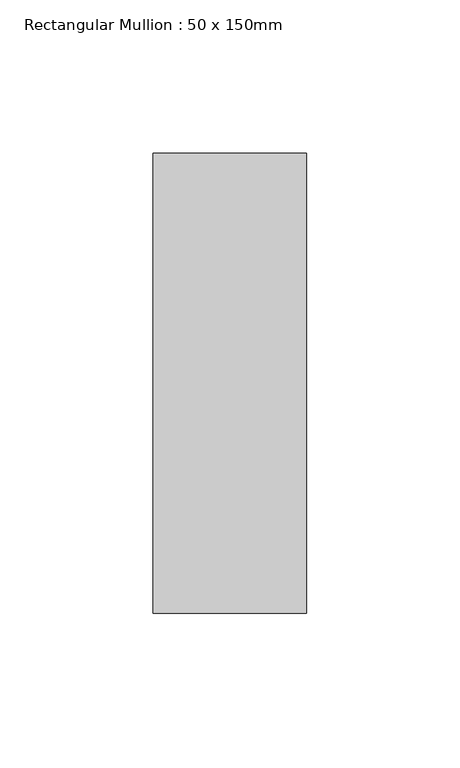
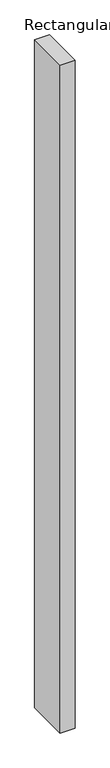
"""IFC4 building model written with IfcOpenShell, lengths in millimetres: member geometry, Rectangular Mullion : 50 x 150mm."""

import ifcopenshell
import ifcopenshell.guid

model = None  # the IFC model being written
_history = None  # IfcOwnerHistory: only IFC2X3 demands one
_inside = {}  # id of a spatial element -> (the spatial element, [elements in it])
_under = {}  # id of a project, library or spatial element -> (it, [spatial elements below it])
_declared = {}  # id of a project -> (the project, [libraries it declares])
_typed = {}  # id of a type object -> (the type object, [elements of that type])
_made_of = {}  # id of a material, layer set ... -> (it, [elements and type objects made of it])


def new_model(schema):
    """Start an empty IFC model of exactly this schema.

    Asked for "IFC4X3", IfcOpenShell would pick the latest addendum, in which some entities
    have other attributes; the version numbers below select the first issue.
    IFC2X3 requires an IfcOwnerHistory on every rooted entity: one is made here for all.
    """
    global model, _history
    if schema == "IFC4X3":
        model = ifcopenshell.file(schema_version=(4, 3, 0, 0))
    else:
        model = ifcopenshell.file(schema=schema)
    _inside.clear()
    _under.clear()
    _declared.clear()
    _typed.clear()
    _made_of.clear()
    _history = None
    if model.schema == "IFC2X3":
        org = make("IfcOrganization", Name="unknown")
        user = make(
            "IfcPersonAndOrganization",
            ThePerson=make("IfcPerson", FamilyName="unknown"),
            TheOrganization=org,
        )
        app = make(
            "IfcApplication",
            ApplicationDeveloper=org,
            Version="unknown",
            ApplicationFullName="unknown",
            ApplicationIdentifier="unknown",
        )
        _history = make(
            "IfcOwnerHistory",
            OwningUser=user,
            OwningApplication=app,
            ChangeAction="ADDED",
            CreationDate=0,
        )
    return model


def make(cls, **values):
    """One entity of the class cls with the attributes given. An attribute that is None is left unset."""
    return model.create_entity(
        cls, **{name: value for name, value in values.items() if value is not None}
    )


def rooted(cls, **values):
    """An entity with a GlobalId (a new one), such as an element, a storey or a relation."""
    return make(cls, GlobalId=ifcopenshell.guid.new(), OwnerHistory=_history, **values)


def si_unit(unit_type, name, prefix=None):
    """IfcSIUnit, for example si_unit("LENGTHUNIT", "METRE", prefix="MILLI")."""
    return make("IfcSIUnit", UnitType=unit_type, Prefix=prefix, Name=name)


def assignment(units):
    """IfcUnitAssignment: the units of a project."""
    return None if units is None else make("IfcUnitAssignment", Units=units)


def point(xyz):
    """IfcCartesianPoint."""
    return None if xyz is None else make("IfcCartesianPoint", Coordinates=xyz)


def direction(xyz):
    """IfcDirection."""
    return None if xyz is None else make("IfcDirection", DirectionRatios=xyz)


def frame(location, z_axis=None, x_axis=None):
    """IfcAxis2Placement3D, a coordinate frame: its origin and axes. An axis left out is left unset."""
    return make(
        "IfcAxis2Placement3D",
        Location=point(location),
        Axis=direction(z_axis),
        RefDirection=direction(x_axis),
    )


def origin():
    """The frame at (0, 0, 0) with its axes left unset."""
    return frame((0.0, 0.0, 0.0))


def place(relative_to, where):
    """IfcLocalPlacement: puts the frame where relative to a parent placement (None: the world)."""
    return make(
        "IfcLocalPlacement", PlacementRelTo=relative_to, RelativePlacement=where
    )


def context(
    kind, dimensions, precision=None, world=None, true_north=None, identifier=None
):
    """IfcGeometricRepresentationContext, for example the 3D "Model" context."""
    return make(
        "IfcGeometricRepresentationContext",
        ContextIdentifier=identifier,
        ContextType=kind,
        CoordinateSpaceDimension=dimensions,
        Precision=precision,
        WorldCoordinateSystem=world,
        TrueNorth=true_north,
    )


def project(units=None, contexts=None):
    """IfcProject with its units and contexts."""
    return rooted(
        "IfcProject",
        Name="project",
        RepresentationContexts=contexts,
        UnitsInContext=assignment(units),
    )


def spatial(cls, under=None, at=None, **own):
    """A site, building, storey or space (cls), placed at a placement, below another one or the project."""
    s = rooted(cls, ObjectPlacement=at, **own)
    if under is not None:
        _under.setdefault(under.id(), (under, []))[1].append(s)
    return s


def polyline(points):
    """IfcPolyline through the points."""
    return make("IfcPolyline", Points=[point(p) for p in points])


def outline(outer, holes=None, kind="AREA"):
    """IfcArbitraryClosedProfileDef: a profile drawn as a closed curve; with holes, ...WithVoids."""
    if holes is None:
        return make("IfcArbitraryClosedProfileDef", ProfileType=kind, OuterCurve=outer)
    return make(
        "IfcArbitraryProfileDefWithVoids",
        ProfileType=kind,
        OuterCurve=outer,
        InnerCurves=holes,
    )


def extrude(swept, where, along, depth):
    """IfcExtrudedAreaSolid: the profile swept, set in the frame where, extruded along a direction by depth."""
    return make(
        "IfcExtrudedAreaSolid",
        SweptArea=swept,
        Position=where,
        ExtrudedDirection=direction(along),
        Depth=depth,
    )


def shape(context_of_items, identifier, shape_type, items):
    """IfcShapeRepresentation: the items that make up one representation, for example the "Body"."""
    return make(
        "IfcShapeRepresentation",
        ContextOfItems=context_of_items,
        RepresentationIdentifier=identifier,
        RepresentationType=shape_type,
        Items=items,
    )


def source(mapping_origin, context_of_items, identifier, shape_type, items):
    """IfcRepresentationMap: a shape defined once, which mapped items show again and again."""
    return make(
        "IfcRepresentationMap",
        MappingOrigin=mapping_origin,
        MappedRepresentation=shape(context_of_items, identifier, shape_type, items),
    )


def transform(
    local_origin,
    x_axis=None,
    y_axis=None,
    z_axis=None,
    scale=None,
    scale2=None,
    scale3=None,
    uniform=True,
):
    """IfcCartesianTransformationOperator3D, or its non-uniform kind. x_axis, y_axis, z_axis: its Axis1, 2, 3."""
    if uniform:
        return make(
            "IfcCartesianTransformationOperator3D",
            Axis1=direction(x_axis),
            Axis2=direction(y_axis),
            LocalOrigin=point(local_origin),
            Scale=scale,
            Axis3=direction(z_axis),
        )
    return make(
        "IfcCartesianTransformationOperator3DnonUniform",
        Axis1=direction(x_axis),
        Axis2=direction(y_axis),
        LocalOrigin=point(local_origin),
        Scale=scale,
        Axis3=direction(z_axis),
        Scale2=scale2,
        Scale3=scale3,
    )


def mapped(mapping_source, mapping_target):
    """IfcMappedItem: shows the shape of a source again, moved by a transform."""
    return make(
        "IfcMappedItem", MappingSource=mapping_source, MappingTarget=mapping_target
    )


def made_of(thing, what):
    """Note that an element or type object is made of a material, layer set ...; save() writes the relation."""
    if what is not None:
        _made_of.setdefault(what.id(), (what, []))[1].append(thing)
    return thing


def element(
    cls,
    number,
    at=None,
    inside=None,
    cuts=None,
    type_object=None,
    material=None,
    context=None,
    identifier="Body",
    shape_type=None,
    held_by="IfcProductDefinitionShape",
    body=None,
    shapes=None,
    **own,
):
    """One element of the class cls, such as IfcWall. Its Tag is "e" and its number.

    at: its placement. inside: the storey or other place that contains it. cuts: it is an
    opening in that element (IfcRelVoidsElement). A single representation is given by context,
    identifier, shape_type and body (its items); several are given by shapes. held_by: the class
    of the entity that holds the representations. save() writes the other relations.
    """
    e = rooted(cls, Tag="e%d" % number, ObjectPlacement=at, **own)
    if body is not None:
        shapes = [shape(context, identifier, shape_type, body)]
    if shapes is not None:
        e.Representation = make(held_by, Representations=shapes)
    if inside is not None:
        _inside.setdefault(inside.id(), (inside, []))[1].append(e)
    if cuts is not None:
        rooted(
            "IfcRelVoidsElement", RelatingBuildingElement=cuts, RelatedOpeningElement=e
        )
    if type_object is not None:
        _typed.setdefault(type_object.id(), (type_object, []))[1].append(e)
    return made_of(e, material)


def aggregate(whole, parts):
    """IfcRelAggregates: a whole, such as a stair, and the parts it consists of."""
    return rooted("IfcRelAggregates", RelatingObject=whole, RelatedObjects=parts)


def save(model, path):
    """Write the relations noted so far, then the file.

    IfcRelAggregates (storeys below a building ...), IfcRelContainedInSpatialStructure (elements
    in a storey), IfcRelDefinesByType, IfcRelAssociatesMaterial and IfcRelDeclares: one each for
    every whole, place, type object, material and project.
    """
    for whole, parts in _under.values():
        aggregate(whole, parts)
    for where, things in _inside.values():
        rooted(
            "IfcRelContainedInSpatialStructure",
            RelatedElements=things,
            RelatingStructure=where,
        )
    for kind, things in _typed.values():
        rooted("IfcRelDefinesByType", RelatedObjects=things, RelatingType=kind)
    for what, things in _made_of.values():
        rooted("IfcRelAssociatesMaterial", RelatedObjects=things, RelatingMaterial=what)
    for by, libraries in _declared.values():
        rooted("IfcRelDeclares", RelatingContext=by, RelatedDefinitions=libraries)
    model.write(path)


def rectangular_mullion_50_x_150mm_6225e4e3(model_context):
    return source(origin(), model_context, "Body", "SweptSolid", [
        extrude(outline(polyline([(25.0, 75.0), (25.0, -75.0), (-25.0, -75.0), (-25.0, 75.0), (25.0, 75.0)])), frame((0.0, 0.0, -2400.0), z_axis=(0.0, 0.0, 1.0), x_axis=(1.0, 0.0, 0.0)), (0.0, 0.0, 1.0), 2400.0),
    ])


if __name__ == "__main__":
    model = new_model("IFC4")
    model_context = context("Model", 3, world=origin())
    ifc_project = project(units=[si_unit("LENGTHUNIT", "METRE", prefix="MILLI")], contexts=[model_context])
    site = spatial("IfcSite", under=ifc_project)
    building = spatial("IfcBuilding", under=site)
    placement = place(None, origin())
    rectangular_mullion_50_x_150mm_shape = rectangular_mullion_50_x_150mm_6225e4e3(model_context)
    element("IfcMember", 1, ObjectType="Rectangular Mullion : 50 x 150mm", at=placement, inside=building, context=model_context, shape_type="MappedRepresentation", body=[
        mapped(rectangular_mullion_50_x_150mm_shape, transform((0.0, 0.0, 0.0), x_axis=(1.0, 0.0, 0.0), y_axis=(0.0, 1.0, 0.0), z_axis=(0.0, 0.0, 1.0))),
    ])
    save(model, "model.ifc")

# Revit data of these elements
# Type "Rectangular Mullion : 50 x 150mm"
#   built-in parameter 1007304 = 0.492126 (stored number, unit not read)
#   built-in parameter 1007301 = 0.082021 (stored number, unit not read)
#   built-in parameter 1007300 = 0.082021 (stored number, unit not read)
# Element 1 (IfcMember, "Rectangular Mullion : 50 x 150mm")
#   Materials on its faces: "Aluminium"
# Materials
#   "Aluminium": class "Metal", colour RGB 247 247 247, transparency 0, Description = "Aluminium 6061", Cost = 0
